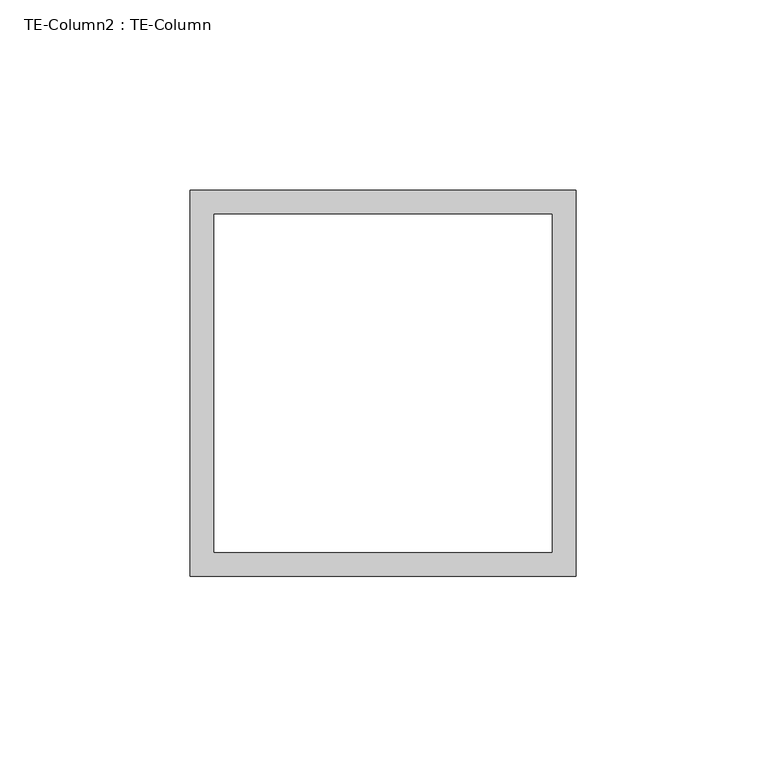
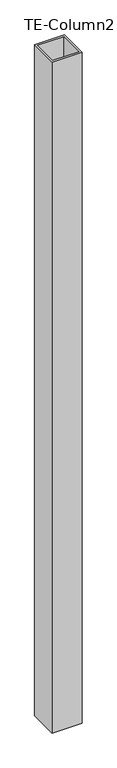
"""IFC4 building model written with IfcOpenShell, lengths in millimetres: proxy geometry, TE-Column2 : TE-Column."""

from ifc_helpers import new_model, si_unit, frame, origin, place, context, project, spatial, polyline, outline, extrude, source, transform, mapped, element, save


def te_column2_te_column_b03e1283(model_context):
    return source(origin(), model_context, "Body", "SweptSolid", [
        extrude(outline(polyline([(590318.6434739, -531667.7913841), (590318.6434739, -531769.3913841), (590217.0434739, -531769.3913841), (590217.0434739, -531667.7913841), (590318.6434739, -531667.7913841)]), holes=[polyline([(590223.3934739, -531674.1413841), (590223.3934739, -531763.0413841), (590312.2934739, -531763.0413841), (590312.2934739, -531674.1413841), (590223.3934739, -531674.1413841)])]), frame((0.0, 0.0, 28.575), z_axis=(0.0, 0.0, 1.0), x_axis=(1.0, 0.0, 0.0)), (0.0, 0.0, 1.0), 2406.65),
    ])


if __name__ == "__main__":
    model = new_model("IFC4")
    model_context = context("Model", 3, world=origin())
    ifc_project = project(units=[si_unit("LENGTHUNIT", "METRE", prefix="MILLI")], contexts=[model_context])
    site = spatial("IfcSite", under=ifc_project)
    building = spatial("IfcBuilding", under=site)
    placement = place(None, origin())
    te_column2_te_column_shape = te_column2_te_column_b03e1283(model_context)
    element("IfcBuildingElementProxy", 1, Name="TE-Column2 : TE-Column", ObjectType="TE-Column2 : TE-Column", at=placement, inside=building, context=model_context, shape_type="MappedRepresentation", body=[
        mapped(te_column2_te_column_shape, transform((0.0, 0.0, 0.0), x_axis=(1.0, 0.0, 0.0), y_axis=(0.0, 1.0, 0.0), z_axis=(0.0, 0.0, 1.0))),
    ])
    save(model, "model.ifc")

# Revit data of these elements
# Element 1 (IfcBuildingElementProxy, "TE-Column2 : TE-Column")
#   Materials on its faces: "4\"X4\" GALV. HSS TUBING"
# Materials
#   "4\"X4\" GALV. HSS TUBING": class "Generic", colour RGB 211 211 207, transparency 0, Cost = 0
